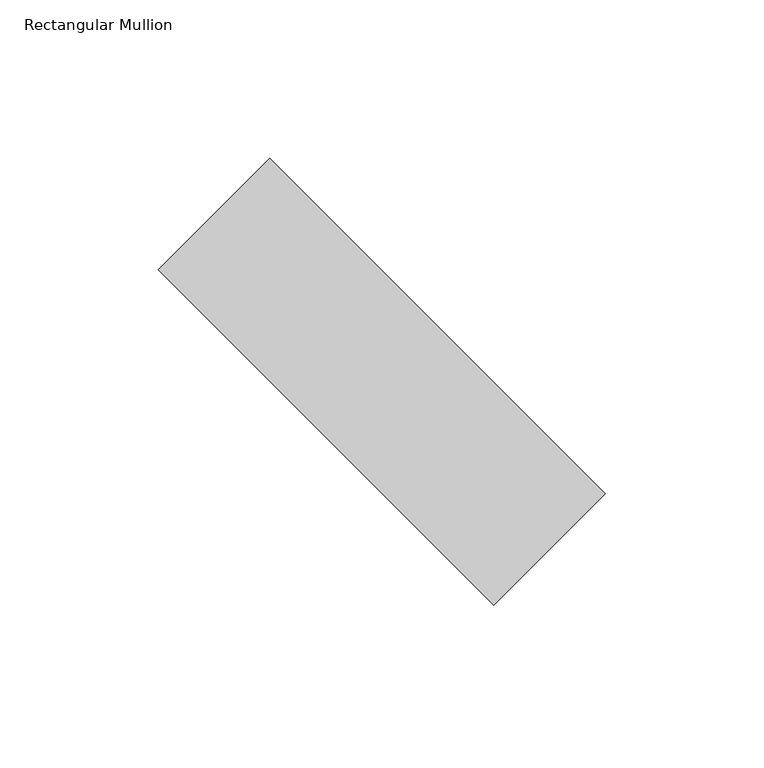
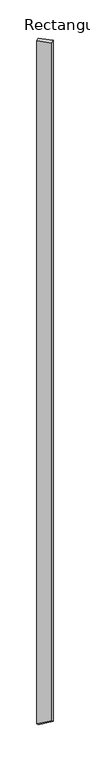
"""IFC4 building model written with IfcOpenShell, lengths in millimetres: member geometry, Rectangular Mullion : tilted mullions."""

import ifcopenshell
import ifcopenshell.guid

model = None  # the IFC model being written
_history = None  # IfcOwnerHistory: only IFC2X3 demands one
_inside = {}  # id of a spatial element -> (the spatial element, [elements in it])
_under = {}  # id of a project, library or spatial element -> (it, [spatial elements below it])
_declared = {}  # id of a project -> (the project, [libraries it declares])
_typed = {}  # id of a type object -> (the type object, [elements of that type])
_made_of = {}  # id of a material, layer set ... -> (it, [elements and type objects made of it])


def new_model(schema):
    """Start an empty IFC model of exactly this schema.

    Asked for "IFC4X3", IfcOpenShell would pick the latest addendum, in which some entities
    have other attributes; the version numbers below select the first issue.
    IFC2X3 requires an IfcOwnerHistory on every rooted entity: one is made here for all.
    """
    global model, _history
    if schema == "IFC4X3":
        model = ifcopenshell.file(schema_version=(4, 3, 0, 0))
    else:
        model = ifcopenshell.file(schema=schema)
    _inside.clear()
    _under.clear()
    _declared.clear()
    _typed.clear()
    _made_of.clear()
    _history = None
    if model.schema == "IFC2X3":
        org = make("IfcOrganization", Name="unknown")
        user = make(
            "IfcPersonAndOrganization",
            ThePerson=make("IfcPerson", FamilyName="unknown"),
            TheOrganization=org,
        )
        app = make(
            "IfcApplication",
            ApplicationDeveloper=org,
            Version="unknown",
            ApplicationFullName="unknown",
            ApplicationIdentifier="unknown",
        )
        _history = make(
            "IfcOwnerHistory",
            OwningUser=user,
            OwningApplication=app,
            ChangeAction="ADDED",
            CreationDate=0,
        )
    return model


def make(cls, **values):
    """One entity of the class cls with the attributes given. An attribute that is None is left unset."""
    return model.create_entity(
        cls, **{name: value for name, value in values.items() if value is not None}
    )


def rooted(cls, **values):
    """An entity with a GlobalId (a new one), such as an element, a storey or a relation."""
    return make(cls, GlobalId=ifcopenshell.guid.new(), OwnerHistory=_history, **values)


def si_unit(unit_type, name, prefix=None):
    """IfcSIUnit, for example si_unit("LENGTHUNIT", "METRE", prefix="MILLI")."""
    return make("IfcSIUnit", UnitType=unit_type, Prefix=prefix, Name=name)


def assignment(units):
    """IfcUnitAssignment: the units of a project."""
    return None if units is None else make("IfcUnitAssignment", Units=units)


def point(xyz):
    """IfcCartesianPoint."""
    return None if xyz is None else make("IfcCartesianPoint", Coordinates=xyz)


def direction(xyz):
    """IfcDirection."""
    return None if xyz is None else make("IfcDirection", DirectionRatios=xyz)


def frame(location, z_axis=None, x_axis=None):
    """IfcAxis2Placement3D, a coordinate frame: its origin and axes. An axis left out is left unset."""
    return make(
        "IfcAxis2Placement3D",
        Location=point(location),
        Axis=direction(z_axis),
        RefDirection=direction(x_axis),
    )


def origin():
    """The frame at (0, 0, 0) with its axes left unset."""
    return frame((0.0, 0.0, 0.0))


def place(relative_to, where):
    """IfcLocalPlacement: puts the frame where relative to a parent placement (None: the world)."""
    return make(
        "IfcLocalPlacement", PlacementRelTo=relative_to, RelativePlacement=where
    )


def context(
    kind, dimensions, precision=None, world=None, true_north=None, identifier=None
):
    """IfcGeometricRepresentationContext, for example the 3D "Model" context."""
    return make(
        "IfcGeometricRepresentationContext",
        ContextIdentifier=identifier,
        ContextType=kind,
        CoordinateSpaceDimension=dimensions,
        Precision=precision,
        WorldCoordinateSystem=world,
        TrueNorth=true_north,
    )


def project(units=None, contexts=None):
    """IfcProject with its units and contexts."""
    return rooted(
        "IfcProject",
        Name="project",
        RepresentationContexts=contexts,
        UnitsInContext=assignment(units),
    )


def spatial(cls, under=None, at=None, **own):
    """A site, building, storey or space (cls), placed at a placement, below another one or the project."""
    s = rooted(cls, ObjectPlacement=at, **own)
    if under is not None:
        _under.setdefault(under.id(), (under, []))[1].append(s)
    return s


def faces_of(points, faces, orient=None, outer=None):
    """IfcFace entities. A face is a list of loops; a loop is a list of indices into points, from 0.

    orient and outer hold one flag for each loop. By default every Orientation is true, the
    first loop of a face is its IfcFaceOuterBound and the others are IfcFaceBound.
    """
    made = []
    for i, loops in enumerate(faces):
        bounds = []
        for j, loop in enumerate(loops):
            is_outer = j == 0 if outer is None else outer[i][j]
            bounds.append(
                make(
                    "IfcFaceOuterBound" if is_outer else "IfcFaceBound",
                    Bound=make("IfcPolyLoop", Polygon=[points[k] for k in loop]),
                    Orientation=True if orient is None else orient[i][j],
                )
            )
        made.append(make("IfcFace", Bounds=bounds))
    return made


def faceted_brep(points, faces, orient=None, outer=None, voids=None):
    """IfcFacetedBrep: a solid bounded by flat faces; with voids (closed shells), ...WithVoids."""
    shared = [point(p) for p in points]
    hull = make("IfcClosedShell", CfsFaces=faces_of(shared, faces, orient, outer))
    if voids is None:
        return make("IfcFacetedBrep", Outer=hull)
    return make(
        "IfcFacetedBrepWithVoids",
        Outer=hull,
        Voids=[
            make(cls, CfsFaces=faces_of(shared, fs, o, b)) for cls, fs, o, b in voids
        ],
    )


def shape(context_of_items, identifier, shape_type, items):
    """IfcShapeRepresentation: the items that make up one representation, for example the "Body"."""
    return make(
        "IfcShapeRepresentation",
        ContextOfItems=context_of_items,
        RepresentationIdentifier=identifier,
        RepresentationType=shape_type,
        Items=items,
    )


def source(mapping_origin, context_of_items, identifier, shape_type, items):
    """IfcRepresentationMap: a shape defined once, which mapped items show again and again."""
    return make(
        "IfcRepresentationMap",
        MappingOrigin=mapping_origin,
        MappedRepresentation=shape(context_of_items, identifier, shape_type, items),
    )


def transform(
    local_origin,
    x_axis=None,
    y_axis=None,
    z_axis=None,
    scale=None,
    scale2=None,
    scale3=None,
    uniform=True,
):
    """IfcCartesianTransformationOperator3D, or its non-uniform kind. x_axis, y_axis, z_axis: its Axis1, 2, 3."""
    if uniform:
        return make(
            "IfcCartesianTransformationOperator3D",
            Axis1=direction(x_axis),
            Axis2=direction(y_axis),
            LocalOrigin=point(local_origin),
            Scale=scale,
            Axis3=direction(z_axis),
        )
    return make(
        "IfcCartesianTransformationOperator3DnonUniform",
        Axis1=direction(x_axis),
        Axis2=direction(y_axis),
        LocalOrigin=point(local_origin),
        Scale=scale,
        Axis3=direction(z_axis),
        Scale2=scale2,
        Scale3=scale3,
    )


def mapped(mapping_source, mapping_target):
    """IfcMappedItem: shows the shape of a source again, moved by a transform."""
    return make(
        "IfcMappedItem", MappingSource=mapping_source, MappingTarget=mapping_target
    )


def made_of(thing, what):
    """Note that an element or type object is made of a material, layer set ...; save() writes the relation."""
    if what is not None:
        _made_of.setdefault(what.id(), (what, []))[1].append(thing)
    return thing


def element(
    cls,
    number,
    at=None,
    inside=None,
    cuts=None,
    type_object=None,
    material=None,
    context=None,
    identifier="Body",
    shape_type=None,
    held_by="IfcProductDefinitionShape",
    body=None,
    shapes=None,
    **own,
):
    """One element of the class cls, such as IfcWall. Its Tag is "e" and its number.

    at: its placement. inside: the storey or other place that contains it. cuts: it is an
    opening in that element (IfcRelVoidsElement). A single representation is given by context,
    identifier, shape_type and body (its items); several are given by shapes. held_by: the class
    of the entity that holds the representations. save() writes the other relations.
    """
    e = rooted(cls, Tag="e%d" % number, ObjectPlacement=at, **own)
    if body is not None:
        shapes = [shape(context, identifier, shape_type, body)]
    if shapes is not None:
        e.Representation = make(held_by, Representations=shapes)
    if inside is not None:
        _inside.setdefault(inside.id(), (inside, []))[1].append(e)
    if cuts is not None:
        rooted(
            "IfcRelVoidsElement", RelatingBuildingElement=cuts, RelatedOpeningElement=e
        )
    if type_object is not None:
        _typed.setdefault(type_object.id(), (type_object, []))[1].append(e)
    return made_of(e, material)


def aggregate(whole, parts):
    """IfcRelAggregates: a whole, such as a stair, and the parts it consists of."""
    return rooted("IfcRelAggregates", RelatingObject=whole, RelatedObjects=parts)


def save(model, path):
    """Write the relations noted so far, then the file.

    IfcRelAggregates (storeys below a building ...), IfcRelContainedInSpatialStructure (elements
    in a storey), IfcRelDefinesByType, IfcRelAssociatesMaterial and IfcRelDeclares: one each for
    every whole, place, type object, material and project.
    """
    for whole, parts in _under.values():
        aggregate(whole, parts)
    for where, things in _inside.values():
        rooted(
            "IfcRelContainedInSpatialStructure",
            RelatedElements=things,
            RelatingStructure=where,
        )
    for kind, things in _typed.values():
        rooted("IfcRelDefinesByType", RelatedObjects=things, RelatingType=kind)
    for what, things in _made_of.values():
        rooted("IfcRelAssociatesMaterial", RelatedObjects=things, RelatingMaterial=what)
    for by, libraries in _declared.values():
        rooted("IfcRelDeclares", RelatingContext=by, RelatedDefinitions=libraries)
    model.write(path)


def rectangular_mullion_2c8bbd53(model_context):
    return source(origin(), model_context, "Body", "Brep", [
        faceted_brep([(-35.3553391, 70.7106781, 0.0), (-70.7106781, 35.3553391, 0.0), (35.3553391, -70.7106781, 0.0), (70.7106781, -35.3553391, 0.0), (-35.3553391, 70.7106781, -8054.3689422), (-70.7106781, 35.3553391, -8009.3419618), (35.3553391, -70.7106781, -7944.1258646), (70.7106781, -35.3553391, -7989.152845)], [[[0, 1, 2, 3]], [[1, 0, 4, 5]], [[2, 1, 5, 6]], [[3, 2, 6, 7]], [[0, 3, 7, 4]], [[4, 7, 6, 5]]]),
    ])


if __name__ == "__main__":
    model = new_model("IFC4")
    model_context = context("Model", 3, world=origin())
    ifc_project = project(units=[si_unit("LENGTHUNIT", "METRE", prefix="MILLI")], contexts=[model_context])
    site = spatial("IfcSite", under=ifc_project)
    building = spatial("IfcBuilding", under=site)
    placement = place(None, origin())
    rectangular_mullion_shape = rectangular_mullion_2c8bbd53(model_context)
    element("IfcMember", 1, ObjectType="Rectangular Mullion : tilted mullions", at=placement, inside=building, context=model_context, shape_type="MappedRepresentation", body=[
        mapped(rectangular_mullion_shape, transform((0.0, 0.0, 0.0), x_axis=(1.0, 0.0, 0.0), y_axis=(0.0, 1.0, 0.0), z_axis=(0.0, 0.0, 1.0))),
    ])
    save(model, "model.ifc")

# Revit data of these elements
# Type "Rectangular Mullion : tilted mullions"
#   built-in parameter 1007304 = 0.492126 (stored number, unit not read)
#   built-in parameter 1007301 = 0.082021 (stored number, unit not read)
#   built-in parameter 1007300 = 0.082021 (stored number, unit not read)
# Element 1 (IfcMember, "Rectangular Mullion : tilted mullions")
#   Materials on its faces: "Aluminum"
# Materials
#   "Aluminum": class "Metal", colour RGB 244 244 244, transparency 0, Description = "Aluminum 6061", Cost = 0
